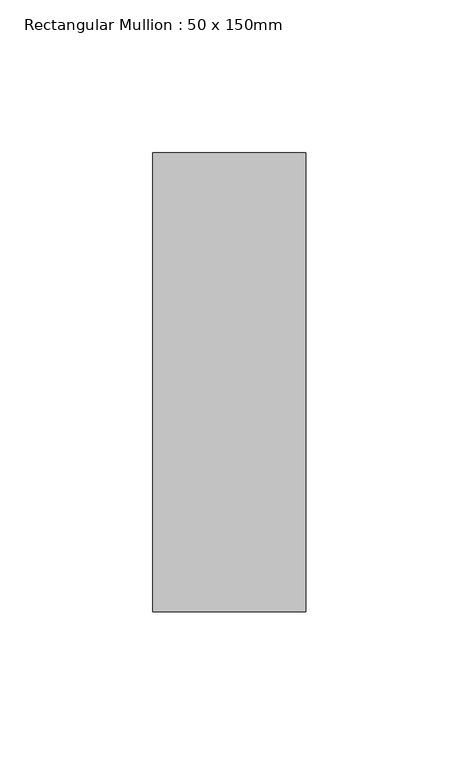
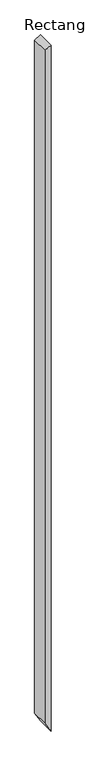
"""IFC4 building model written with IfcOpenShell, lengths in millimetres: member geometry, Rectangular Mullion : 50 x 150mm."""

import ifcopenshell
import ifcopenshell.guid

model = None  # the IFC model being written
_history = None  # IfcOwnerHistory: only IFC2X3 demands one
_inside = {}  # id of a spatial element -> (the spatial element, [elements in it])
_under = {}  # id of a project, library or spatial element -> (it, [spatial elements below it])
_declared = {}  # id of a project -> (the project, [libraries it declares])
_typed = {}  # id of a type object -> (the type object, [elements of that type])
_made_of = {}  # id of a material, layer set ... -> (it, [elements and type objects made of it])


def new_model(schema):
    """Start an empty IFC model of exactly this schema.

    Asked for "IFC4X3", IfcOpenShell would pick the latest addendum, in which some entities
    have other attributes; the version numbers below select the first issue.
    IFC2X3 requires an IfcOwnerHistory on every rooted entity: one is made here for all.
    """
    global model, _history
    if schema == "IFC4X3":
        model = ifcopenshell.file(schema_version=(4, 3, 0, 0))
    else:
        model = ifcopenshell.file(schema=schema)
    _inside.clear()
    _under.clear()
    _declared.clear()
    _typed.clear()
    _made_of.clear()
    _history = None
    if model.schema == "IFC2X3":
        org = make("IfcOrganization", Name="unknown")
        user = make(
            "IfcPersonAndOrganization",
            ThePerson=make("IfcPerson", FamilyName="unknown"),
            TheOrganization=org,
        )
        app = make(
            "IfcApplication",
            ApplicationDeveloper=org,
            Version="unknown",
            ApplicationFullName="unknown",
            ApplicationIdentifier="unknown",
        )
        _history = make(
            "IfcOwnerHistory",
            OwningUser=user,
            OwningApplication=app,
            ChangeAction="ADDED",
            CreationDate=0,
        )
    return model


def make(cls, **values):
    """One entity of the class cls with the attributes given. An attribute that is None is left unset."""
    return model.create_entity(
        cls, **{name: value for name, value in values.items() if value is not None}
    )


def rooted(cls, **values):
    """An entity with a GlobalId (a new one), such as an element, a storey or a relation."""
    return make(cls, GlobalId=ifcopenshell.guid.new(), OwnerHistory=_history, **values)


def si_unit(unit_type, name, prefix=None):
    """IfcSIUnit, for example si_unit("LENGTHUNIT", "METRE", prefix="MILLI")."""
    return make("IfcSIUnit", UnitType=unit_type, Prefix=prefix, Name=name)


def assignment(units):
    """IfcUnitAssignment: the units of a project."""
    return None if units is None else make("IfcUnitAssignment", Units=units)


def point(xyz):
    """IfcCartesianPoint."""
    return None if xyz is None else make("IfcCartesianPoint", Coordinates=xyz)


def direction(xyz):
    """IfcDirection."""
    return None if xyz is None else make("IfcDirection", DirectionRatios=xyz)


def frame(location, z_axis=None, x_axis=None):
    """IfcAxis2Placement3D, a coordinate frame: its origin and axes. An axis left out is left unset."""
    return make(
        "IfcAxis2Placement3D",
        Location=point(location),
        Axis=direction(z_axis),
        RefDirection=direction(x_axis),
    )


def origin():
    """The frame at (0, 0, 0) with its axes left unset."""
    return frame((0.0, 0.0, 0.0))


def place(relative_to, where):
    """IfcLocalPlacement: puts the frame where relative to a parent placement (None: the world)."""
    return make(
        "IfcLocalPlacement", PlacementRelTo=relative_to, RelativePlacement=where
    )


def context(
    kind, dimensions, precision=None, world=None, true_north=None, identifier=None
):
    """IfcGeometricRepresentationContext, for example the 3D "Model" context."""
    return make(
        "IfcGeometricRepresentationContext",
        ContextIdentifier=identifier,
        ContextType=kind,
        CoordinateSpaceDimension=dimensions,
        Precision=precision,
        WorldCoordinateSystem=world,
        TrueNorth=true_north,
    )


def project(units=None, contexts=None):
    """IfcProject with its units and contexts."""
    return rooted(
        "IfcProject",
        Name="project",
        RepresentationContexts=contexts,
        UnitsInContext=assignment(units),
    )


def spatial(cls, under=None, at=None, **own):
    """A site, building, storey or space (cls), placed at a placement, below another one or the project."""
    s = rooted(cls, ObjectPlacement=at, **own)
    if under is not None:
        _under.setdefault(under.id(), (under, []))[1].append(s)
    return s


def polyline(points):
    """IfcPolyline through the points."""
    return make("IfcPolyline", Points=[point(p) for p in points])


def outline(outer, holes=None, kind="AREA"):
    """IfcArbitraryClosedProfileDef: a profile drawn as a closed curve; with holes, ...WithVoids."""
    if holes is None:
        return make("IfcArbitraryClosedProfileDef", ProfileType=kind, OuterCurve=outer)
    return make(
        "IfcArbitraryProfileDefWithVoids",
        ProfileType=kind,
        OuterCurve=outer,
        InnerCurves=holes,
    )


def extrude(swept, where, along, depth):
    """IfcExtrudedAreaSolid: the profile swept, set in the frame where, extruded along a direction by depth."""
    return make(
        "IfcExtrudedAreaSolid",
        SweptArea=swept,
        Position=where,
        ExtrudedDirection=direction(along),
        Depth=depth,
    )


def shape(context_of_items, identifier, shape_type, items):
    """IfcShapeRepresentation: the items that make up one representation, for example the "Body"."""
    return make(
        "IfcShapeRepresentation",
        ContextOfItems=context_of_items,
        RepresentationIdentifier=identifier,
        RepresentationType=shape_type,
        Items=items,
    )


def source(mapping_origin, context_of_items, identifier, shape_type, items):
    """IfcRepresentationMap: a shape defined once, which mapped items show again and again."""
    return make(
        "IfcRepresentationMap",
        MappingOrigin=mapping_origin,
        MappedRepresentation=shape(context_of_items, identifier, shape_type, items),
    )


def transform(
    local_origin,
    x_axis=None,
    y_axis=None,
    z_axis=None,
    scale=None,
    scale2=None,
    scale3=None,
    uniform=True,
):
    """IfcCartesianTransformationOperator3D, or its non-uniform kind. x_axis, y_axis, z_axis: its Axis1, 2, 3."""
    if uniform:
        return make(
            "IfcCartesianTransformationOperator3D",
            Axis1=direction(x_axis),
            Axis2=direction(y_axis),
            LocalOrigin=point(local_origin),
            Scale=scale,
            Axis3=direction(z_axis),
        )
    return make(
        "IfcCartesianTransformationOperator3DnonUniform",
        Axis1=direction(x_axis),
        Axis2=direction(y_axis),
        LocalOrigin=point(local_origin),
        Scale=scale,
        Axis3=direction(z_axis),
        Scale2=scale2,
        Scale3=scale3,
    )


def mapped(mapping_source, mapping_target):
    """IfcMappedItem: shows the shape of a source again, moved by a transform."""
    return make(
        "IfcMappedItem", MappingSource=mapping_source, MappingTarget=mapping_target
    )


def made_of(thing, what):
    """Note that an element or type object is made of a material, layer set ...; save() writes the relation."""
    if what is not None:
        _made_of.setdefault(what.id(), (what, []))[1].append(thing)
    return thing


def element(
    cls,
    number,
    at=None,
    inside=None,
    cuts=None,
    type_object=None,
    material=None,
    context=None,
    identifier="Body",
    shape_type=None,
    held_by="IfcProductDefinitionShape",
    body=None,
    shapes=None,
    **own,
):
    """One element of the class cls, such as IfcWall. Its Tag is "e" and its number.

    at: its placement. inside: the storey or other place that contains it. cuts: it is an
    opening in that element (IfcRelVoidsElement). A single representation is given by context,
    identifier, shape_type and body (its items); several are given by shapes. held_by: the class
    of the entity that holds the representations. save() writes the other relations.
    """
    e = rooted(cls, Tag="e%d" % number, ObjectPlacement=at, **own)
    if body is not None:
        shapes = [shape(context, identifier, shape_type, body)]
    if shapes is not None:
        e.Representation = make(held_by, Representations=shapes)
    if inside is not None:
        _inside.setdefault(inside.id(), (inside, []))[1].append(e)
    if cuts is not None:
        rooted(
            "IfcRelVoidsElement", RelatingBuildingElement=cuts, RelatedOpeningElement=e
        )
    if type_object is not None:
        _typed.setdefault(type_object.id(), (type_object, []))[1].append(e)
    return made_of(e, material)


def aggregate(whole, parts):
    """IfcRelAggregates: a whole, such as a stair, and the parts it consists of."""
    return rooted("IfcRelAggregates", RelatingObject=whole, RelatedObjects=parts)


def save(model, path):
    """Write the relations noted so far, then the file.

    IfcRelAggregates (storeys below a building ...), IfcRelContainedInSpatialStructure (elements
    in a storey), IfcRelDefinesByType, IfcRelAssociatesMaterial and IfcRelDeclares: one each for
    every whole, place, type object, material and project.
    """
    for whole, parts in _under.values():
        aggregate(whole, parts)
    for where, things in _inside.values():
        rooted(
            "IfcRelContainedInSpatialStructure",
            RelatedElements=things,
            RelatingStructure=where,
        )
    for kind, things in _typed.values():
        rooted("IfcRelDefinesByType", RelatedObjects=things, RelatingType=kind)
    for what, things in _made_of.values():
        rooted("IfcRelAssociatesMaterial", RelatedObjects=things, RelatingMaterial=what)
    for by, libraries in _declared.values():
        rooted("IfcRelDeclares", RelatingContext=by, RelatedDefinitions=libraries)
    model.write(path)


def rectangular_mullion_50_x_150mm_f412d67c(model_context):
    return source(origin(), model_context, "Body", "SweptSolid", [
        extrude(outline(polyline([(0.0, 0.0), (-29.3010691, -50.0), (-5992.1456409, -50.0), (-6077.4667599, 0.0), (0.0, 0.0)])), frame((0.0, -75.0, 0.0), z_axis=(0.0, 1.0, 0.0), x_axis=(0.0, 0.0, 1.0)), (0.0, 0.0, 1.0), 150.0),
    ])


if __name__ == "__main__":
    model = new_model("IFC4")
    model_context = context("Model", 3, world=origin())
    ifc_project = project(units=[si_unit("LENGTHUNIT", "METRE", prefix="MILLI")], contexts=[model_context])
    site = spatial("IfcSite", under=ifc_project)
    building = spatial("IfcBuilding", under=site)
    placement = place(None, origin())
    rectangular_mullion_50_x_150mm_shape = rectangular_mullion_50_x_150mm_f412d67c(model_context)
    element("IfcMember", 1, ObjectType="Rectangular Mullion : 50 x 150mm", at=placement, inside=building, context=model_context, shape_type="MappedRepresentation", body=[
        mapped(rectangular_mullion_50_x_150mm_shape, transform((0.0, 0.0, 0.0), x_axis=(1.0, 0.0, 0.0), y_axis=(0.0, 1.0, 0.0), z_axis=(0.0, 0.0, 1.0))),
    ])
    save(model, "model.ifc")

# Revit data of these elements
# Type "Rectangular Mullion : 50 x 150mm"
#   built-in parameter 1007304 = 0.492126 (stored number, unit not read)
#   built-in parameter 1007301 = 0.082021 (stored number, unit not read)
#   built-in parameter 1007300 = 0.082021 (stored number, unit not read)
# Element 1 (IfcMember, "Rectangular Mullion : 50 x 150mm")
#   Materials on its faces: "Metal - Aluminium"
# Materials
#   "Metal - Aluminium": class "Metal", colour RGB 247 247 247, transparency 0
